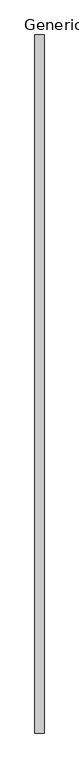
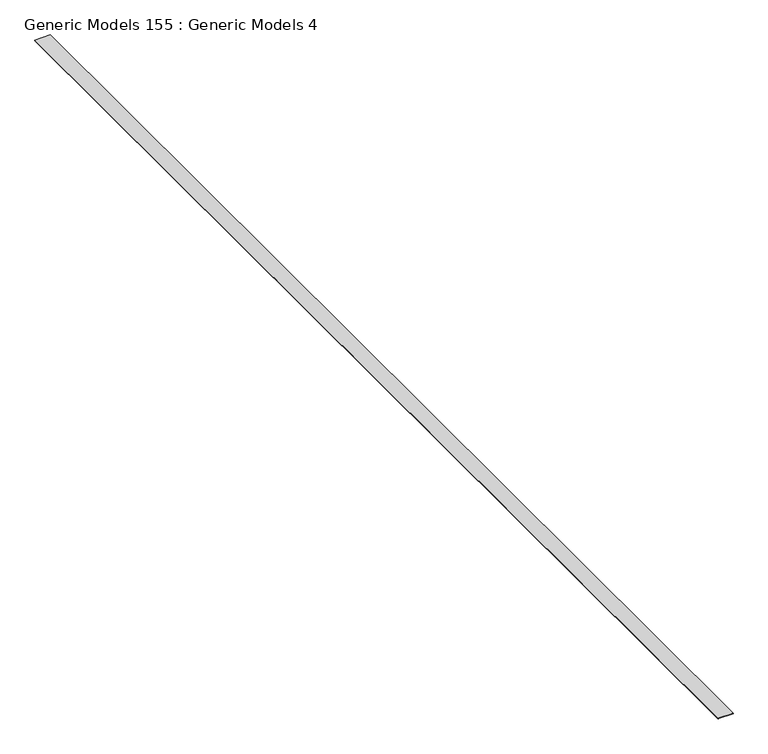
"""IFC4 building model written with IfcOpenShell, lengths in millimetres: proxy geometry, Generic Models 155 : Generic Models 4."""

from ifc_helpers import new_model, si_unit, frame, origin, place, context, project, spatial, polyline, outline, extrude, source, transform, mapped, element, save


def generic_models_155_generic_models_4_4c06f935(model_context):
    return source(origin(), model_context, "Body", "SweptSolid", [
        extrude(outline(polyline([(-6503.7484477, -5493.3230338), (-6606.9079316, -5493.3230338), (-6606.9079316, 2393.3769662), (-6503.7484477, 2393.3769662), (-6503.7484477, -5493.3230338)])), frame((0.0, 0.0, 123263.8963316), z_axis=(0.0, 0.0, 1.0), x_axis=(1.0, 0.0, 0.0)), (0.0, 0.0, 1.0), 1.3753749),
        extrude(outline(polyline([(-6503.7484477, -5493.3230338), (-6606.9079316, -5493.3230338), (-6606.9079316, 2393.3769662), (-6503.7484477, 2393.3769662), (-6503.7484477, -5493.3230338)])), frame((0.0, 0.0, 123260.5026733), z_axis=(0.0, 0.0, 1.0), x_axis=(1.0, 0.0, 0.0)), (0.0, 0.0, 1.0), 1.3753749),
    ])


if __name__ == "__main__":
    model = new_model("IFC4")
    model_context = context("Model", 3, world=origin())
    ifc_project = project(units=[si_unit("LENGTHUNIT", "METRE", prefix="MILLI")], contexts=[model_context])
    site = spatial("IfcSite", under=ifc_project)
    building = spatial("IfcBuilding", under=site)
    placement = place(None, origin())
    generic_models_155_generic_models_4_shape = generic_models_155_generic_models_4_4c06f935(model_context)
    element("IfcBuildingElementProxy", 1, Name="Generic Models 155 : Generic Models 4", ObjectType="Generic Models 155 : Generic Models 4", at=placement, inside=building, context=model_context, shape_type="MappedRepresentation", body=[
        mapped(generic_models_155_generic_models_4_shape, transform((0.0, 0.0, 0.0), x_axis=(1.0, 0.0, 0.0), y_axis=(0.0, 1.0, 0.0), z_axis=(0.0, 0.0, 1.0))),
    ])
    save(model, "model.ifc")

# Revit data of these elements
# Element 1 (IfcBuildingElementProxy, "Generic Models 155 : Generic Models 4")
#   Materials on its faces: "_BED OF SEALANT (ABOVE/BELOW FLASHING)"
# Materials
#   "_BED OF SEALANT (ABOVE/BELOW FLASHING)": class "Generic", colour RGB 253 192 103, transparency 0, Cost = 0
